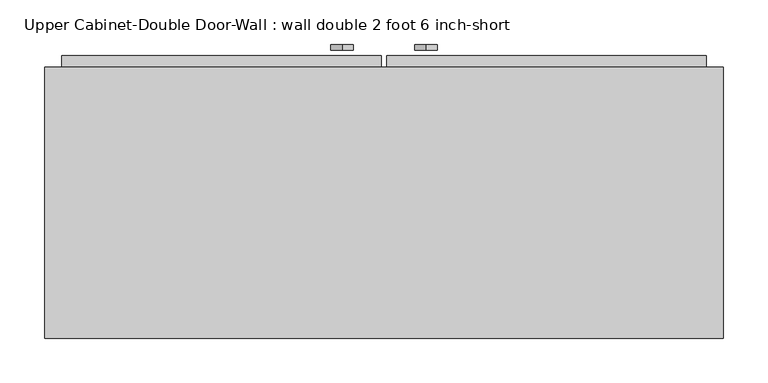
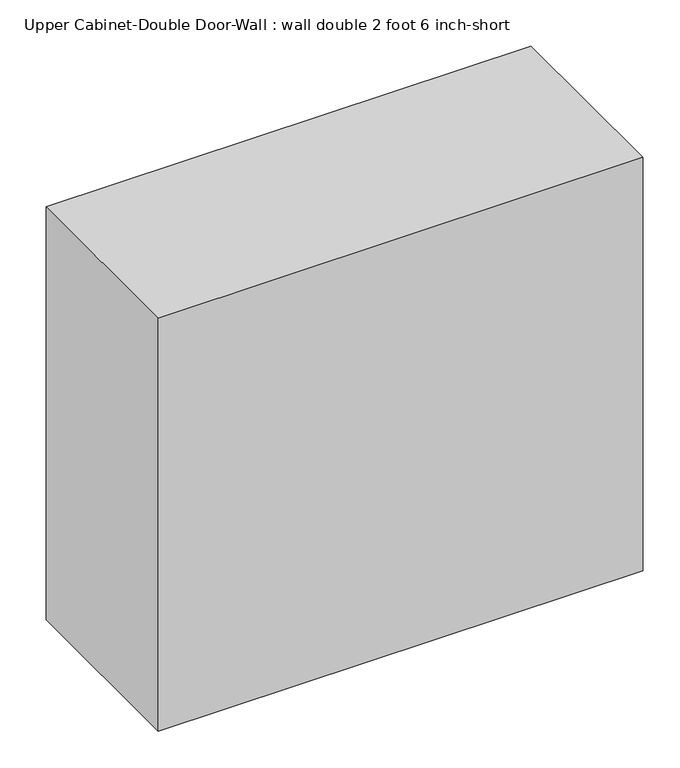
"""IFC4 building model written with IfcOpenShell, lengths in millimetres: furniture geometry, Upper Cabinet-Double Door-Wall : wall double 2 foot 6 inch-short."""

from ifc_helpers import new_model, si_unit, point, frame, frame_2d, origin, place, context, project, spatial, polyline, circle_curve, trimmed, segment, composite_curve, outline, extrude, faceted_brep, source, transform, mapped, element, save


def upper_cabinet_double_door_wall_wall_double_2_foot_6_inch_f6462eeb(model_context):
    return source(origin(), model_context, "Body", "SolidModel", [
        faceted_brep([(-351.2288372, 56.35625, 2133.6), (-351.2288372, 56.35625, 1447.8), (410.7711628, 56.35625, 1447.8), (410.7711628, 56.35625, 2133.6), (-351.2288372, 361.15625, 2133.6), (410.7711628, 361.15625, 2133.6), (410.7711628, 361.15625, 1447.8), (-351.2288372, 361.15625, 1447.8), (-332.1788372, 361.15625, 2114.55), (-332.1788372, 361.15625, 1466.85), (391.7211628, 361.15625, 1466.85), (391.7211628, 361.15625, 2114.55), (391.7211628, 75.40625, 2114.55), (-332.1788372, 75.40625, 2114.55), (391.7211628, 75.40625, 1466.85), (-332.1788372, 75.40625, 1466.85)], [[[0, 1, 2, 3]], [[4, 5, 6, 7], [8, 9, 10, 11]], [[1, 0, 4, 7]], [[2, 1, 7, 6]], [[3, 2, 6, 5]], [[0, 3, 5, 4]], [[8, 11, 12, 13]], [[11, 10, 14, 12]], [[10, 9, 15, 14]], [[9, 8, 13, 15]], [[13, 12, 14, 15]]]),
        extrude(outline(polyline([(32.9461628, 373.85625), (391.7211628, 373.85625), (391.7211628, 342.10625), (32.9461628, 342.10625), (32.9461628, 373.85625)])), frame((0.0, 0.0, 1466.85), z_axis=(0.0, 0.0, 1.0), x_axis=(1.0, 0.0, 0.0)), (0.0, 0.0, 1.0), 647.7),
        extrude(outline(polyline([(-332.1788372, 373.85625), (26.5961628, 373.85625), (26.5961628, 342.10625), (-332.1788372, 342.10625), (-332.1788372, 373.85625)])), frame((0.0, 0.0, 1466.85), z_axis=(0.0, 0.0, 1.0), x_axis=(1.0, 0.0, 0.0)), (0.0, 0.0, 1.0), 647.7),
        extrude(outline(composite_curve([segment(trimmed(circle_curve(frame_2d((1610.0214732, 76.8007051)), 12.7), [point((1597.3214732, 76.8007051))], [point((1622.7214732, 76.8007051))], False, "CARTESIAN"), True, "CONTINUOUS"), segment(trimmed(circle_curve(frame_2d((1610.0214732, 76.8007051)), 12.7), [point((1622.7214732, 76.8007051))], [point((1597.3214732, 76.8007051))], False, "CARTESIAN"), True, "CONTINUOUS")], self_intersect=False)), frame((0.0, 380.20625, 0.0), z_axis=(0.0, 1.0, 0.0), x_axis=(0.0, 0.0, 1.0)), (0.0, 0.0, 1.0), 6.35),
        extrude(outline(composite_curve([segment(trimmed(circle_curve(frame_2d((1610.0214732, -17.2583796)), 12.7), [point((1597.3214732, -17.2583796))], [point((1622.7214732, -17.2583796))], False, "CARTESIAN"), True, "CONTINUOUS"), segment(trimmed(circle_curve(frame_2d((1610.0214732, -17.2583796)), 12.7), [point((1622.7214732, -17.2583796))], [point((1597.3214732, -17.2583796))], False, "CARTESIAN"), True, "CONTINUOUS")], self_intersect=False)), frame((0.0, 380.20625, 0.0), z_axis=(0.0, 1.0, 0.0), x_axis=(0.0, 0.0, 1.0)), (0.0, 0.0, 1.0), 6.35),
    ])


if __name__ == "__main__":
    model = new_model("IFC4")
    model_context = context("Model", 3, world=origin())
    ifc_project = project(units=[si_unit("LENGTHUNIT", "METRE", prefix="MILLI")], contexts=[model_context])
    site = spatial("IfcSite", under=ifc_project)
    building = spatial("IfcBuilding", under=site)
    placement = place(None, origin())
    upper_cabinet_double_door_wall_wall_double_2_foot_6_inch_shape = upper_cabinet_double_door_wall_wall_double_2_foot_6_inch_f6462eeb(model_context)
    element("IfcFurniture", 1, ObjectType="Upper Cabinet-Double Door-Wall : wall double 2 foot 6 inch-short", at=placement, inside=building, context=model_context, shape_type="MappedRepresentation", body=[
        mapped(upper_cabinet_double_door_wall_wall_double_2_foot_6_inch_shape, transform((0.0, 0.0, 0.0), x_axis=(1.0, 0.0, 0.0), y_axis=(0.0, 1.0, 0.0), z_axis=(0.0, 0.0, 1.0))),
    ])
    save(model, "model.ifc")

# Revit data of these elements
# Type "Upper Cabinet-Double Door-Wall : wall double 2 foot 6 inch-short"
#   Assembly Code = "C1030410"
#   Depth = 1' - 0"
#   Height = 2' - 3"
#   Top Of Cabinet = 7' - 0"
#   Width = 2' - 6"
#   Cabinet Material = Base cabinet 2120100 Aspekt - 83012120100 - White
#   Door/Drawer Material = Base cabinet 2120100 Aspekt - 83012120100 - White
#   Handle Material = Cabinets - Handles
#   Default Elevation = 0
# Element 1 (IfcFurniture, "Upper Cabinet-Double Door-Wall : wall double 2 foot 6 inch-short")
#   Materials on its faces: "Base cabinet 2120100 Aspekt - 83012120100 - White"
# Materials
#   "Base cabinet 2120100 Aspekt - 83012120100 - White": class "Miscellaneous", colour RGB 255 255 255, transparency 0, Manufacturer = "Marbodal", URL = "http://www.marbodal.se", Cost = 0
#   "Cabinets - Handles": class "Metal", colour RGB 57 57 57, transparency 0
